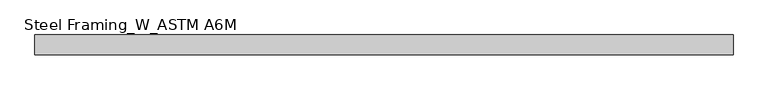
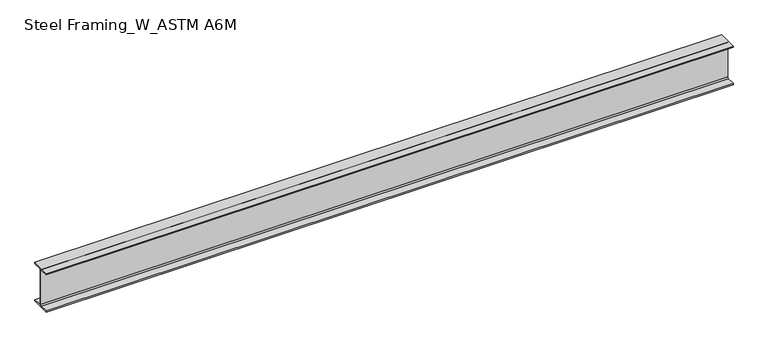
"""IFC4 building model written with IfcOpenShell, lengths in millimetres: beam geometry, Steel Framing_W_ASTM A6M : H_SB_AR_S02_W360x51_RB2."""

from ifc_helpers import new_model, si_unit, point, frame, frame_2d, origin, place, context, project, spatial, polyline, circle_curve, trimmed, segment, composite_curve, outline, extrude, source, transform, mapped, element, save


def steel_framing_w_astm_a6m_8694913f(model_context):
    return source(origin(), model_context, "Body", "SweptSolid", [
        extrude(outline(composite_curve([segment(polyline([(85.5, -166.4), (85.5, -178.0), (-85.5, -178.0), (-85.5, -166.4), (-13.72, -166.4)]), True, "CONTINUOUS"), segment(trimmed(circle_curve(frame_2d((-13.72, -156.3)), 10.1), [point((-13.72, -166.4))], [point((-3.62, -156.3))], True, "CARTESIAN"), True, "CONTINUOUS"), segment(polyline([(-3.62, -156.3), (-3.62, 156.3)]), True, "CONTINUOUS"), segment(trimmed(circle_curve(frame_2d((-13.72, 156.3)), 10.1), [point((-3.62, 156.3))], [point((-13.72, 166.4))], True, "CARTESIAN"), True, "CONTINUOUS"), segment(polyline([(-13.72, 166.4), (-85.5, 166.4), (-85.5, 178.0), (85.5, 178.0), (85.5, 166.4), (13.72, 166.4)]), True, "CONTINUOUS"), segment(trimmed(circle_curve(frame_2d((13.72, 156.3)), 10.1), [point((13.72, 166.4))], [point((3.62, 156.3))], True, "CARTESIAN"), True, "CONTINUOUS"), segment(polyline([(3.62, 156.3), (3.62, -156.3)]), True, "CONTINUOUS"), segment(trimmed(circle_curve(frame_2d((13.72, -156.3)), 10.1), [point((3.62, -156.3))], [point((13.72, -166.4))], True, "CARTESIAN"), True, "CONTINUOUS"), segment(polyline([(13.72, -166.4), (85.5, -166.4)]), True, "CONTINUOUS")], self_intersect=False)), frame((-3014.95, 0.0, 0.0), z_axis=(1.0, 0.0, 0.0), x_axis=(0.0, 1.0, 0.0)), (0.0, 0.0, 1.0), 6017.2),
    ])


if __name__ == "__main__":
    model = new_model("IFC4")
    model_context = context("Model", 3, world=origin())
    ifc_project = project(units=[si_unit("LENGTHUNIT", "METRE", prefix="MILLI")], contexts=[model_context])
    site = spatial("IfcSite", under=ifc_project)
    building = spatial("IfcBuilding", under=site)
    placement = place(None, origin())
    steel_framing_w_astm_a6m_shape = steel_framing_w_astm_a6m_8694913f(model_context)
    element("IfcBeam", 1, ObjectType="Steel Framing_W_ASTM A6M : H_SB_AR_S02_W360x51_RB2", at=placement, inside=building, context=model_context, shape_type="MappedRepresentation", body=[
        mapped(steel_framing_w_astm_a6m_shape, transform((0.0, 0.0, 0.0), x_axis=(1.0, 0.0, 0.0), y_axis=(0.0, 1.0, 0.0), z_axis=(0.0, 0.0, 1.0))),
    ])
    save(model, "model.ifc")

# Revit data of these elements
# Type "Steel Framing_W_ASTM A6M : H_SB_AR_S02_W360x51_RB2"
#   Type Mark = "RB2"
#   Section Name Key = "W14x34"
#   Width = 17.1 cm
#   Web Thickness = 0.724 cm
#   Web Fillet = 1.01 cm
#   Warping Constant = 287000.0 cm⁶
#   Torsional Moment of Inertia = 23.70 cm⁴
#   Section Area = 64.5 cm²
#   Plastic Modulus weak axis = 174.0 cm³
#   Plastic Modulus strong axis = 895.0 cm³
#   Perimeter = 1.36 m²/m
#   Nominal Weight = 51.00 kgf/m
#   Moment of Inertia weak axis = 970.00 cm⁴
#   Moment of Inertia strong axis = 14200.00 cm⁴
#   Height = 35.6 cm
#   Flange Thickness = 1.16 cm
#   Elastic Modulus weak axis = 113.0 cm³
#   Elastic Modulus strong axis = 796.0 cm³
#   Centroid Vertical = 17.8 cm
#   Centroid Horizontal = 8.55 cm
#   Length [instance default] = 1500 mm
#   Structural Material [instance default] = Steel, 45-345
#   Bolt Spacing = 0
#   Assembly Code = ""
# Element 1 (IfcBeam, "Steel Framing_W_ASTM A6M : H_SB_AR_S02_W360x51_RB2")
#   Materials on its faces: "Steel, 45-345"
# Materials
#   "Steel, 45-345": class "Metal", colour RGB 189 187 185, transparency 0, Description = "Steel 345 MPa", Cost = 0
